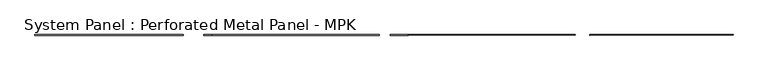
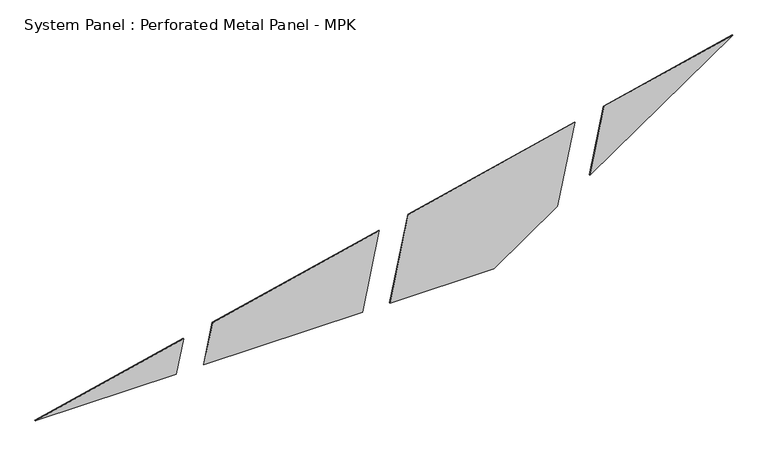
"""IFC4 building model written with IfcOpenShell, lengths in millimetres: plate geometry, System Panel : Perforated Metal Panel - MPK."""

from ifc_helpers import new_model, si_unit, frame, origin, place, context, project, spatial, polyline, outline, extrude, source, transform, mapped, element, save


def system_panel_perforated_metal_panel_mpk_086f5f12(model_context):
    return source(origin(), model_context, "Body", "SweptSolid", [
        extrude(outline(polyline([(0.0, -12024.4566539), (0.0, -7157.0389313), (1197.5335563, -6906.8588907), (0.0, -12024.4566539)])), frame((0.0, 0.0, 0.0), z_axis=(0.0, 1.0, 0.0), x_axis=(0.0, 0.0, 1.0)), (0.0, 0.0, 1.0), 20.0),
        extrude(outline(polyline([(0.0, -6209.3045392), (0.0, -740.9792912), (2776.0803661, -161.0206795), (1430.7051889, -5910.4119692), (0.0, -6209.3045392)])), frame((0.0, 0.0, 0.0), z_axis=(0.0, 1.0, 0.0), x_axis=(0.0, 0.0, 1.0)), (0.0, 0.0, 1.0), 20.0),
        extrude(outline(polyline([(0.0, 206.7551009), (0.0, 3785.5599023), (1505.4449194, 5989.5870023), (4354.627176, 6584.8175317), (3009.2519988, 835.426242), (0.0, 206.7551009)])), frame((0.0, 0.0, 0.0), z_axis=(0.0, 1.0, 0.0), x_axis=(0.0, 0.0, 1.0)), (0.0, 0.0, 1.0), 20.0),
        extrude(outline(polyline([(4587.7988086, 7581.2644532), (2260.5370002, 7095.0697652), (5627.519397, 12024.4566539), (4587.7988086, 7581.2644532)])), frame((0.0, 0.0, 0.0), z_axis=(0.0, 1.0, 0.0), x_axis=(0.0, 0.0, 1.0)), (0.0, 0.0, 1.0), 20.0),
    ])


if __name__ == "__main__":
    model = new_model("IFC4")
    model_context = context("Model", 3, world=origin())
    ifc_project = project(units=[si_unit("LENGTHUNIT", "METRE", prefix="MILLI")], contexts=[model_context])
    site = spatial("IfcSite", under=ifc_project)
    building = spatial("IfcBuilding", under=site)
    placement = place(None, origin())
    system_panel_perforated_metal_panel_mpk_shape = system_panel_perforated_metal_panel_mpk_086f5f12(model_context)
    element("IfcPlate", 1, ObjectType="System Panel : Perforated Metal Panel - MPK", at=placement, inside=building, context=model_context, shape_type="MappedRepresentation", body=[
        mapped(system_panel_perforated_metal_panel_mpk_shape, transform((0.0, 0.0, 0.0), x_axis=(1.0, 0.0, 0.0), y_axis=(0.0, 1.0, 0.0), z_axis=(0.0, 0.0, 1.0))),
    ])
    save(model, "model.ifc")

# Revit data of these elements
# Element 1 (IfcPlate, "System Panel : Perforated Metal Panel - MPK")
#   Materials on its faces: "Perforated  Metal Panels - MPK"
# Materials
#   "Perforated  Metal Panels - MPK": class "Miscellaneous", colour RGB 127 127 127, transparency 0
